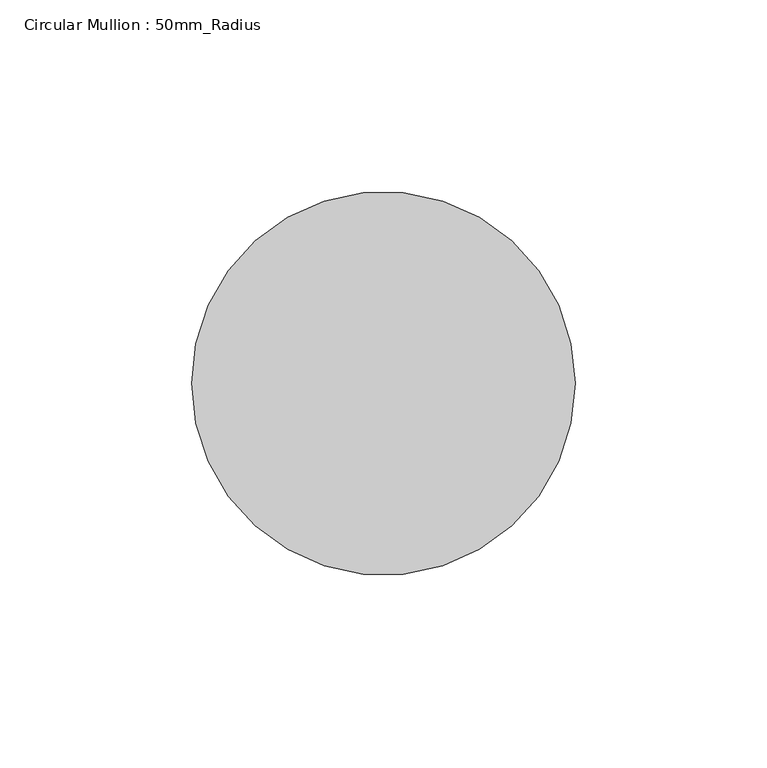
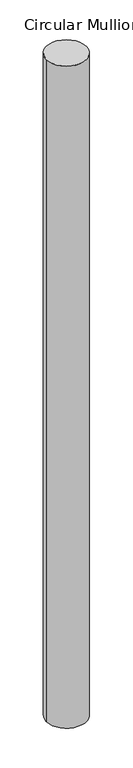
"""IFC4 building model written with IfcOpenShell, lengths in millimetres: member geometry, Circular Mullion : 50mm_Radius."""

from ifc_helpers import new_model, si_unit, point, frame, origin, origin_2d, place, context, project, spatial, circle_curve, trimmed, segment, composite_curve, outline, extrude, source, transform, mapped, element, save


def circular_mullion_50mm_radius_298adcc5(model_context):
    return source(origin(), model_context, "Body", "SweptSolid", [
        extrude(outline(composite_curve([segment(trimmed(circle_curve(origin_2d(), 50.0), [point((50.0, 0.0))], [point((-50.0, 0.0))], False, "CARTESIAN"), True, "CONTINUOUS"), segment(trimmed(circle_curve(origin_2d(), 50.0), [point((-50.0, 0.0))], [point((50.0, 0.0))], False, "CARTESIAN"), True, "CONTINUOUS")], self_intersect=False)), frame((0.0, 0.0, -1755.0000003), z_axis=(0.0, 0.0, 1.0), x_axis=(1.0, 0.0, 0.0)), (0.0, 0.0, 1.0), 1755.0000003),
    ])


if __name__ == "__main__":
    model = new_model("IFC4")
    model_context = context("Model", 3, world=origin())
    ifc_project = project(units=[si_unit("LENGTHUNIT", "METRE", prefix="MILLI")], contexts=[model_context])
    site = spatial("IfcSite", under=ifc_project)
    building = spatial("IfcBuilding", under=site)
    placement = place(None, origin())
    circular_mullion_50mm_radius_shape = circular_mullion_50mm_radius_298adcc5(model_context)
    element("IfcMember", 1, ObjectType="Circular Mullion : 50mm_Radius", at=placement, inside=building, context=model_context, shape_type="MappedRepresentation", body=[
        mapped(circular_mullion_50mm_radius_shape, transform((0.0, 0.0, 0.0), x_axis=(1.0, 0.0, 0.0), y_axis=(0.0, 1.0, 0.0), z_axis=(0.0, 0.0, 1.0))),
    ])
    save(model, "model.ifc")

# Revit data of these elements
# Type "Circular Mullion : 50mm_Radius"
#   Keynote = "H11"
#   built-in parameter 1007350 = 0.164042 (stored number, unit not read)
# Element 1 (IfcMember, "Circular Mullion : 50mm_Radius")
#   Materials on its faces: "Aluminium"
# Materials
#   "Aluminium": class "Metal", colour RGB 247 247 247, transparency 0, Description = "Aluminium 6061", Cost = 0
